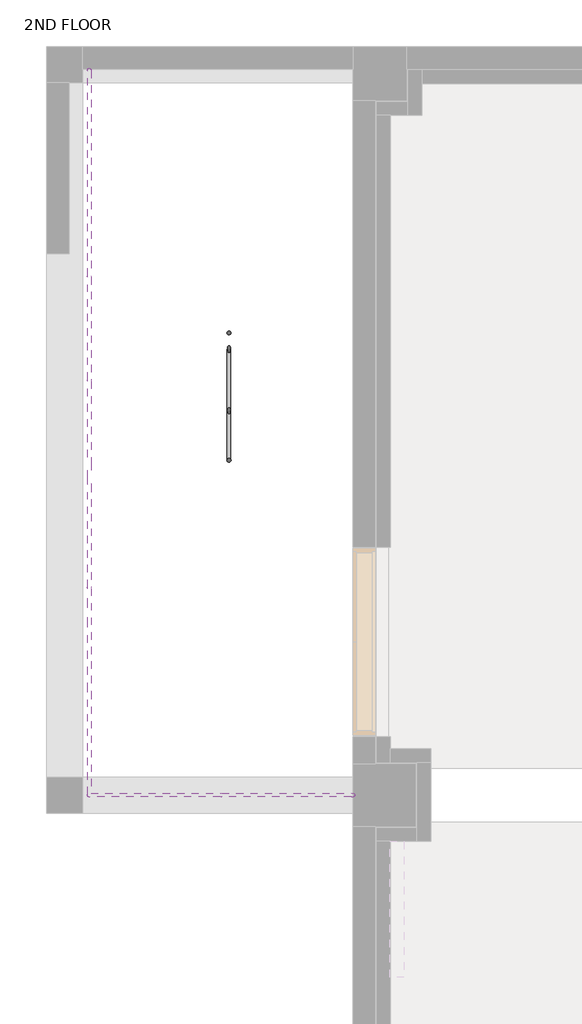
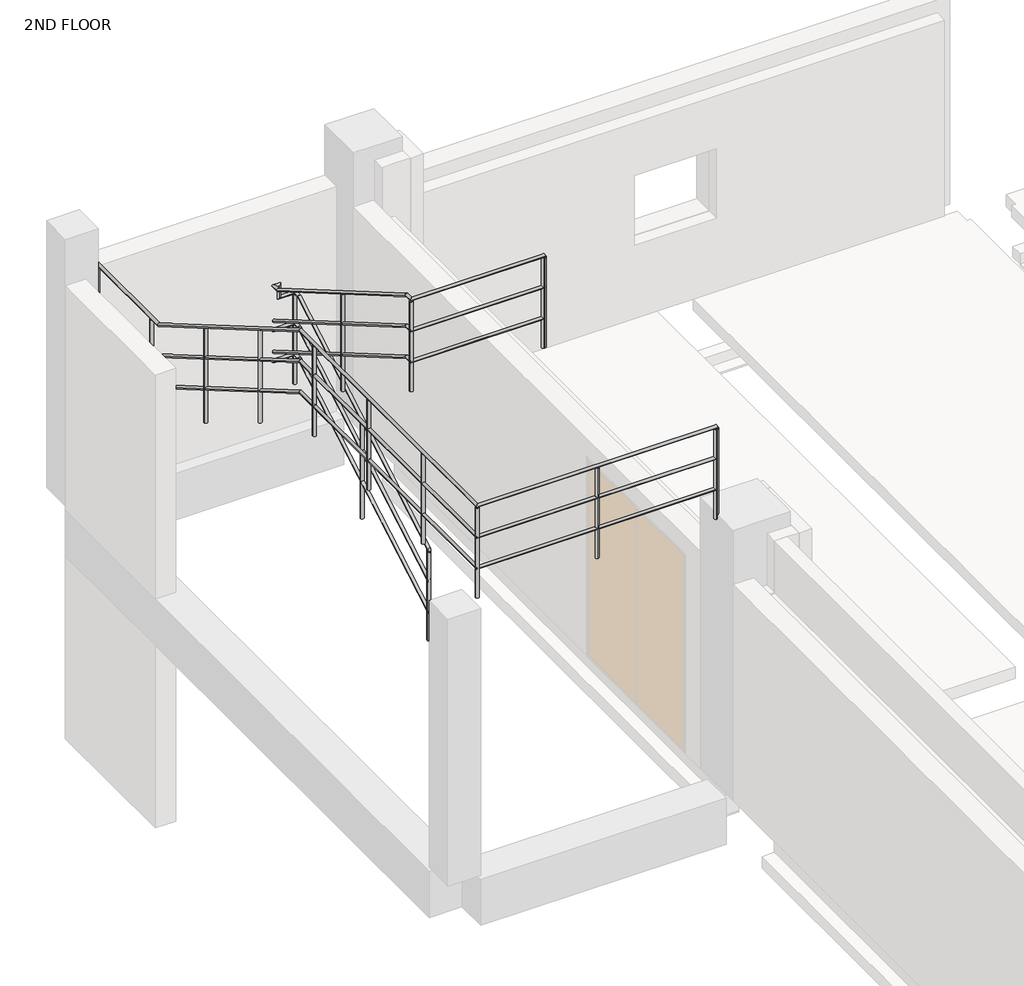
# One storey, part 6 of 7: 2 railings.
"""IFC4 building model written with IfcOpenShell, lengths in millimetres."""

from ifc_helpers import new_model, si_unit, point, frame, frame_2d, origin, place, context, project, spatial, circle_curve, ellipse_curve, trimmed, segment, composite_curve, outline, extrude, element, save
from ifc_brep_helpers import plane_surface, cylinder_surface, advanced_brep

model = new_model("IFC4")

# Units and contexts
model_context = context("Model", 3, world=origin())
ifc_project = project(units=[si_unit("LENGTHUNIT", "METRE", prefix="MILLI")], contexts=[model_context])

# Site, building, storey
site = spatial("IfcSite", under=ifc_project)
building = spatial("IfcBuilding", under=site)
storey = spatial("IfcBuildingStorey", under=building, Name="2ND FLOOR", Elevation=10600.0)

# Railings
placement = place(None, origin())
element("IfcRailing", 1, ObjectType="H_RL_AR_S10_Steel Handrail_H1200_STAIR", at=placement, inside=storey, context=model_context, shape_type="SolidModel", body=[
    advanced_brep(
    [(-1656.0, -4300.0, 11873.8369637), (-1694.0, -4300.0, 11873.8369637), (-1656.0, -1544.8633663, 13481.0), (-1694.0, -1544.8633663, 13481.0), (-1906.0, -1531.1366337, 13642.0), (-1944.0, -1531.1366337, 13642.0), (-1944.0, -4255.1366337, 15231.0), (-1906.0, -4255.1366337, 15231.0), (-1656.0, -1431.0, 13481.0), (-1694.0, -1469.0, 13481.0), (-1868.0, -1431.0, 13481.0), (-1868.0, -1469.0, 13481.0), (-1868.0, -1431.0, 13642.0), (-1868.0, -1469.0, 13642.0), (-1944.0, -1431.0, 13642.0), (-1906.0, -1469.0, 13642.0), (-1944.0, -4369.0, 15231.0), (-1906.0, -4331.0, 15231.0), (-300.0, -4369.0, 15231.0), (-300.0, -4331.0, 15231.0)],
    [
        (0, 1, ellipse_curve(frame((-1675.0, -4300.0, 11873.8369637), z_axis=(0.0, -1.0, 0.0), x_axis=(0.0, 0.0, -1.0)), 21.9963696, 19.0)),
        (1, 0, ellipse_curve(frame((-1675.0, -4300.0, 11873.8369637), z_axis=(0.0, -1.0, 0.0), x_axis=(0.0, 0.0, -1.0)), 21.9963696, 19.0)),
        (0, 2),
        (2, 3, ellipse_curve(frame((-1675.0, -1544.8633663, 13481.0), z_axis=(0.0, -0.9653442134540491, -0.2609799792144664), x_axis=(0.0, 0.2609799792144666, -0.9653442134540492)), 19.6820986, 19.0)),
        (3, 1),
        (3, 2, ellipse_curve(frame((-1675.0, -1544.8633663, 13481.0), z_axis=(0.0, -0.9653442134540491, -0.2609799792144664), x_axis=(0.0, 0.2609799792144666, -0.9653442134540492)), 19.6820986, 19.0)),
        (4, 5, ellipse_curve(frame((-1925.0, -1531.1366337, 13642.0), z_axis=(0.0, -0.965344213454049, 0.26097997921446664), x_axis=(0.0, -0.2609799792144667, -0.9653442134540489)), 19.6820986, 19.0)),
        (5, 6),
        (6, 7, ellipse_curve(frame((-1925.0, -4255.1366337, 15231.0), z_axis=(0.0, 0.965344213454049, -0.2609799792144667), x_axis=(0.0, -0.26097997921446675, -0.965344213454049)), 19.6820986, 19.0)),
        (7, 4),
        (5, 4, ellipse_curve(frame((-1925.0, -1531.1366337, 13642.0), z_axis=(0.0, -0.965344213454049, 0.26097997921446664), x_axis=(0.0, -0.2609799792144667, -0.9653442134540489)), 19.6820986, 19.0)),
        (7, 6, ellipse_curve(frame((-1925.0, -4255.1366337, 15231.0), z_axis=(0.0, 0.965344213454049, -0.2609799792144667), x_axis=(0.0, -0.26097997921446675, -0.965344213454049)), 19.6820986, 19.0)),
        (2, 8),
        (8, 9, ellipse_curve(frame((-1675.0, -1450.0, 13481.0), z_axis=(0.7071067811865466, -0.7071067811865485, 0.0), x_axis=(-0.7071067811865485, -0.7071067811865466, 0.0)), 26.8700577, 19.0)),
        (9, 3),
        (9, 8, ellipse_curve(frame((-1675.0, -1450.0, 13481.0), z_axis=(0.7071067811865466, -0.7071067811865485, 0.0), x_axis=(-0.7071067811865485, -0.7071067811865466, 0.0)), 26.8700577, 19.0)),
        (8, 10),
        (10, 11, ellipse_curve(frame((-1868.0, -1450.0, 13481.0), z_axis=(0.7071067811865475, 0.0, -0.7071067811865475), x_axis=(0.7071067811865476, 0.0, 0.7071067811865474)), 26.8700577, 19.0)),
        (11, 9),
        (11, 10, ellipse_curve(frame((-1868.0, -1450.0, 13481.0), z_axis=(0.7071067811865475, 0.0, -0.7071067811865475), x_axis=(0.7071067811865476, 0.0, 0.7071067811865474)), 26.8700577, 19.0)),
        (10, 12),
        (12, 13, ellipse_curve(frame((-1868.0, -1450.0, 13642.0), z_axis=(0.7071067811865475, 0.0, -0.7071067811865475), x_axis=(-0.7071067811865474, 0.0, -0.7071067811865476)), 26.8700577, 19.0)),
        (13, 11),
        (13, 12, ellipse_curve(frame((-1868.0, -1450.0, 13642.0), z_axis=(0.7071067811865475, 0.0, -0.7071067811865475), x_axis=(-0.7071067811865474, 0.0, -0.7071067811865476)), 26.8700577, 19.0)),
        (12, 14),
        (14, 15, ellipse_curve(frame((-1925.0, -1450.0, 13642.0), z_axis=(0.7071067811865416, 0.7071067811865536, 0.0), x_axis=(0.7071067811865535, -0.7071067811865417, 0.0)), 26.8700577, 19.0)),
        (15, 13),
        (15, 14, ellipse_curve(frame((-1925.0, -1450.0, 13642.0), z_axis=(0.7071067811865416, 0.7071067811865536, 0.0), x_axis=(0.7071067811865535, -0.7071067811865417, 0.0)), 26.8700577, 19.0)),
        (14, 5),
        (4, 15),
        (6, 16),
        (16, 17, ellipse_curve(frame((-1925.0, -4350.0, 15231.0), z_axis=(-0.7071067811865553, 0.7071067811865396, 0.0), x_axis=(0.7071067811865394, 0.7071067811865556, 0.0)), 26.8700577, 19.0)),
        (17, 7),
        (17, 16, ellipse_curve(frame((-1925.0, -4350.0, 15231.0), z_axis=(-0.7071067811865553, 0.7071067811865396, 0.0), x_axis=(0.7071067811865394, 0.7071067811865556, 0.0)), 26.8700577, 19.0)),
        (18, 19, circle_curve(frame((-300.0, -4350.0, 15231.0), z_axis=(1.0, 0.0, 0.0), x_axis=(0.0, 1.0, 0.0)), 19.0)),
        (19, 18, circle_curve(frame((-300.0, -4350.0, 15231.0), z_axis=(1.0, 0.0, 0.0), x_axis=(0.0, 1.0, 0.0)), 19.0)),
        (16, 18),
        (19, 17),
    ],
    [
        plane_surface(frame((-1675.0, -4300.0, 11895.8333333), z_axis=(0.0, -1.0, 0.0), x_axis=(0.0, 0.0, 1.0))),
        cylinder_surface(frame((-1675.0, -4290.4264505, 11879.4215342), z_axis=(0.0, -0.8637789008984333, -0.5038710255240862), x_axis=(-1.0, 0.0, 0.0)), 19.0),
        cylinder_surface(frame((-1925.0, -1535.5735495, 13644.5882009), z_axis=(0.0, 0.8637789008984331, -0.5038710255240867), x_axis=(1.0, 0.0, 0.0)), 19.0),
        cylinder_surface(frame((-1675.0, -1550.0, 13481.0), z_axis=(0.0, -1.0, 0.0), x_axis=(-1.0, 0.0, 0.0)), 19.0),
        cylinder_surface(frame((-1675.0, -1450.0, 13481.0), z_axis=(1.0, 0.0, 0.0), x_axis=(0.0, -1.0, 0.0)), 19.0),
        cylinder_surface(frame((-1868.0, -1450.0, 13500.0), z_axis=(0.0, 0.0, -1.0), x_axis=(0.0, -1.0, 0.0)), 19.0),
        cylinder_surface(frame((-1849.0, -1450.0, 13642.0), z_axis=(1.0, 0.0, 0.0), x_axis=(0.0, -1.0, 0.0)), 19.0),
        cylinder_surface(frame((-1925.0, -1450.0, 13642.0), z_axis=(0.0, 1.0, 0.0), x_axis=(1.0, 0.0, 0.0)), 19.0),
        cylinder_surface(frame((-1925.0, -4250.0, 15231.0), z_axis=(0.0, 1.0, 0.0), x_axis=(1.0, 0.0, 0.0)), 19.0),
        plane_surface(frame((-300.0, -4350.0, 15250.0), z_axis=(1.0, 0.0, 0.0), x_axis=(0.0, 1.0, 0.0))),
        cylinder_surface(frame((-1925.0, -4350.0, 15231.0), z_axis=(-1.0, 0.0, 0.0), x_axis=(0.0, 1.0, 0.0)), 19.0),
    ],
    [
        (0, [[1, 2]]),
        (1, [[-1, 3, 4, 5]]),
        (1, [[-2, -5, 6, -3]]),
        (2, [[7, 8, 9, 10]]),
        (2, [[11, -10, 12, -8]]),
        (3, [[-4, 13, 14, 15]]),
        (3, [[-6, -15, 16, -13]]),
        (4, [[-14, 17, 18, 19]]),
        (4, [[-16, -19, 20, -17]]),
        (5, [[-18, 21, 22, 23]]),
        (5, [[-20, -23, 24, -21]]),
        (6, [[-22, 25, 26, 27]]),
        (6, [[-24, -27, 28, -25]]),
        (7, [[-26, 29, -7, 30]]),
        (7, [[-28, -30, -11, -29]]),
        (8, [[-9, 31, 32, 33]]),
        (8, [[-12, -33, 34, -31]]),
        (9, [[35, 36]]),
        (10, [[-32, 37, -36, 38]]),
        (10, [[-34, -38, -35, -37]]),
    ],
),
    advanced_brep(
    [(-1656.0, -4300.0, 11073.8369637), (-1694.0, -4300.0, 11073.8369637), (-1656.0, -1544.8633663, 12681.0), (-1694.0, -1544.8633663, 12681.0), (-1656.0, -1431.0, 12681.0), (-1694.0, -1469.0, 12681.0)],
    [
        (0, 1, ellipse_curve(frame((-1675.0, -4300.0, 11073.8369637), z_axis=(0.0, -1.0, 0.0), x_axis=(0.0, 0.0, -1.0)), 21.9963696, 19.0)),
        (1, 0, ellipse_curve(frame((-1675.0, -4300.0, 11073.8369637), z_axis=(0.0, -1.0, 0.0), x_axis=(0.0, 0.0, -1.0)), 21.9963696, 19.0)),
        (0, 2),
        (2, 3, ellipse_curve(frame((-1675.0, -1544.8633663, 12681.0), z_axis=(0.0, -0.9653442134540491, -0.2609799792144664), x_axis=(0.0, 0.2609799792144666, -0.9653442134540492)), 19.6820986, 19.0)),
        (3, 1),
        (3, 2, ellipse_curve(frame((-1675.0, -1544.8633663, 12681.0), z_axis=(0.0, -0.9653442134540491, -0.2609799792144664), x_axis=(0.0, 0.2609799792144666, -0.9653442134540492)), 19.6820986, 19.0)),
        (4, 5, ellipse_curve(frame((-1675.0, -1450.0, 12681.0), z_axis=(-0.7071067811865455, 0.7071067811865496, 0.0), x_axis=(-0.7071067811865496, -0.7071067811865455, 0.0)), 26.8700577, 19.0)),
        (5, 4, ellipse_curve(frame((-1675.0, -1450.0, 12681.0), z_axis=(-0.7071067811865455, 0.7071067811865496, 0.0), x_axis=(-0.7071067811865496, -0.7071067811865455, 0.0)), 26.8700577, 19.0)),
        (2, 4),
        (5, 3),
    ],
    [
        plane_surface(frame((-1675.0, -4300.0, 11095.8333333), z_axis=(0.0, -1.0, 0.0), x_axis=(0.0, 0.0, 1.0))),
        cylinder_surface(frame((-1675.0, -4290.4264505, 11079.4215342), z_axis=(0.0, -0.8637789008984333, -0.5038710255240862), x_axis=(-1.0, 0.0, 0.0)), 19.0),
        plane_surface(frame((-1675.0, -1450.0, 12700.0), z_axis=(-0.7071067811865455, 0.7071067811865496, 0.0), x_axis=(0.7071067811865496, 0.7071067811865455, 0.0))),
        cylinder_surface(frame((-1675.0, -1550.0, 12681.0), z_axis=(0.0, -1.0, 0.0), x_axis=(-1.0, 0.0, 0.0)), 19.0),
    ],
    [
        (0, [[1, 2]]),
        (1, [[-1, 3, 4, 5]]),
        (1, [[-2, -5, 6, -3]]),
        (2, [[7, 8]]),
        (3, [[-4, 9, -8, 10]]),
        (3, [[-6, -10, -7, -9]]),
    ],
),
    advanced_brep(
    [(-1656.0, -1431.0, 12681.0), (-1694.0, -1469.0, 12681.0), (-1950.9853486, -1431.0, 12681.0), (-1918.1617504, -1469.0, 12681.0)],
    [
        (0, 1, ellipse_curve(frame((-1675.0, -1450.0, 12681.0), z_axis=(0.7071067811865455, -0.7071067811865496, 0.0), x_axis=(0.7071067811865496, 0.7071067811865455, 0.0)), 26.8700577, 19.0)),
        (1, 0, ellipse_curve(frame((-1675.0, -1450.0, 12681.0), z_axis=(0.7071067811865455, -0.7071067811865496, 0.0), x_axis=(0.7071067811865496, 0.7071067811865455, 0.0)), 26.8700577, 19.0)),
        (2, 3, ellipse_curve(frame((-1934.5735495, -1450.0, 12681.0), z_axis=(-0.707106781186549, -0.6107839182711431, 0.35629061899150194), x_axis=(0.707106781186546, -0.6107839182711456, 0.35629061899150344)), 26.8700577, 19.0)),
        (3, 2, ellipse_curve(frame((-1934.5735495, -1450.0, 12681.0), z_axis=(-0.707106781186549, -0.6107839182711431, 0.35629061899150194), x_axis=(0.707106781186546, -0.6107839182711456, 0.35629061899150344)), 26.8700577, 19.0)),
        (0, 2),
        (3, 1),
    ],
    [
        plane_surface(frame((-1675.0, -1450.0, 12700.0), z_axis=(0.7071067811865455, -0.7071067811865496, 0.0), x_axis=(0.7071067811865496, 0.7071067811865455, 0.0))),
        plane_surface(frame((-1925.0, -1450.0, 12700.0), z_axis=(-0.7071067811865491, -0.6107839182711432, 0.356290618991502), x_axis=(0.7071067811865461, -0.6107839182711456, 0.3562906189915033))),
        cylinder_surface(frame((-1675.0, -1450.0, 12681.0), z_axis=(1.0, 0.0, 0.0), x_axis=(0.0, -1.0, 0.0)), 19.0),
    ],
    [
        (0, [[1, 2]]),
        (1, [[3, 4]]),
        (2, [[-1, 5, -4, 6]]),
        (2, [[-2, -6, -3, -5]]),
    ],
),
    advanced_brep(
    [(-1944.0, -1443.1617504, 12790.6813181), (-1906.0, -1475.9853486, 12809.828417), (-1944.0, -4255.1366337, 14431.0), (-1906.0, -4255.1366337, 14431.0), (-1944.0, -4369.0, 14431.0), (-1906.0, -4331.0, 14431.0)],
    [
        (0, 1, ellipse_curve(frame((-1925.0, -1459.5735495, 12800.2548675), z_axis=(0.707106781186549, 0.6107839182711431, -0.35629061899150194), x_axis=(-0.7071067811865461, 0.6107839182711466, -0.3562906189915013)), 26.8700577, 19.0)),
        (1, 0, ellipse_curve(frame((-1925.0, -1459.5735495, 12800.2548675), z_axis=(0.707106781186549, 0.6107839182711431, -0.35629061899150194), x_axis=(-0.7071067811865461, 0.6107839182711466, -0.3562906189915013)), 26.8700577, 19.0)),
        (0, 2),
        (2, 3, ellipse_curve(frame((-1925.0, -4255.1366337, 14431.0), z_axis=(0.0, 0.965344213454049, -0.26097997921446664), x_axis=(0.0, -0.2609799792144663, -0.9653442134540491)), 19.6820986, 19.0)),
        (3, 1),
        (3, 2, ellipse_curve(frame((-1925.0, -4255.1366337, 14431.0), z_axis=(0.0, 0.965344213454049, -0.26097997921446664), x_axis=(0.0, -0.2609799792144663, -0.9653442134540491)), 19.6820986, 19.0)),
        (4, 5, ellipse_curve(frame((-1925.0, -4350.0, 14431.0), z_axis=(0.7071067811865476, -0.7071067811865475, 0.0), x_axis=(0.7071067811865475, 0.7071067811865476, 0.0)), 26.8700577, 19.0)),
        (5, 4, ellipse_curve(frame((-1925.0, -4350.0, 14431.0), z_axis=(0.7071067811865476, -0.7071067811865475, 0.0), x_axis=(0.7071067811865475, 0.7071067811865476, 0.0)), 26.8700577, 19.0)),
        (2, 4),
        (5, 3),
    ],
    [
        plane_surface(frame((-1925.0, -1450.0, 12816.6666667), z_axis=(0.7071067811865491, 0.6107839182711432, -0.356290618991502), x_axis=(0.7071067811865461, -0.6107839182711456, 0.3562906189915033))),
        cylinder_surface(frame((-1925.0, -1459.5735495, 12800.2548675), z_axis=(0.0, 0.8637789008984332, -0.5038710255240867), x_axis=(1.0, 0.0, 0.0)), 19.0),
        plane_surface(frame((-1925.0, -4350.0, 14450.0), z_axis=(0.7071067811865476, -0.7071067811865475, 0.0), x_axis=(0.7071067811865475, 0.7071067811865476, 0.0))),
        cylinder_surface(frame((-1925.0, -4250.0, 14431.0), z_axis=(0.0, 1.0, 0.0), x_axis=(1.0, 0.0, 0.0)), 19.0),
    ],
    [
        (0, [[1, 2]]),
        (1, [[-1, 3, 4, 5]]),
        (1, [[-2, -5, 6, -3]]),
        (2, [[7, 8]]),
        (3, [[-4, 9, -8, 10]]),
        (3, [[-6, -10, -7, -9]]),
    ],
),
    advanced_brep(
    [(-1656.0, -4300.0, 11473.8369637), (-1694.0, -4300.0, 11473.8369637), (-1656.0, -1544.8633663, 13081.0), (-1694.0, -1544.8633663, 13081.0), (-1656.0, -1431.0, 13081.0), (-1694.0, -1469.0, 13081.0)],
    [
        (0, 1, ellipse_curve(frame((-1675.0, -4300.0, 11473.8369637), z_axis=(0.0, -1.0, 0.0), x_axis=(0.0, 0.0, -1.0)), 21.9963696, 19.0)),
        (1, 0, ellipse_curve(frame((-1675.0, -4300.0, 11473.8369637), z_axis=(0.0, -1.0, 0.0), x_axis=(0.0, 0.0, -1.0)), 21.9963696, 19.0)),
        (0, 2),
        (2, 3, ellipse_curve(frame((-1675.0, -1544.8633663, 13081.0), z_axis=(0.0, -0.9653442134540491, -0.2609799792144664), x_axis=(0.0, 0.2609799792144666, -0.9653442134540492)), 19.6820986, 19.0)),
        (3, 1),
        (3, 2, ellipse_curve(frame((-1675.0, -1544.8633663, 13081.0), z_axis=(0.0, -0.9653442134540491, -0.2609799792144664), x_axis=(0.0, 0.2609799792144666, -0.9653442134540492)), 19.6820986, 19.0)),
        (4, 5, ellipse_curve(frame((-1675.0, -1450.0, 13081.0), z_axis=(-0.7071067811865455, 0.7071067811865496, 0.0), x_axis=(-0.7071067811865496, -0.7071067811865455, 0.0)), 26.8700577, 19.0)),
        (5, 4, ellipse_curve(frame((-1675.0, -1450.0, 13081.0), z_axis=(-0.7071067811865455, 0.7071067811865496, 0.0), x_axis=(-0.7071067811865496, -0.7071067811865455, 0.0)), 26.8700577, 19.0)),
        (2, 4),
        (5, 3),
    ],
    [
        plane_surface(frame((-1675.0, -4300.0, 11495.8333333), z_axis=(0.0, -1.0, 0.0), x_axis=(0.0, 0.0, 1.0))),
        cylinder_surface(frame((-1675.0, -4290.4264505, 11479.4215342), z_axis=(0.0, -0.8637789008984333, -0.5038710255240862), x_axis=(-1.0, 0.0, 0.0)), 19.0),
        plane_surface(frame((-1675.0, -1450.0, 13100.0), z_axis=(-0.7071067811865455, 0.7071067811865496, 0.0), x_axis=(0.7071067811865496, 0.7071067811865455, 0.0))),
        cylinder_surface(frame((-1675.0, -1550.0, 13081.0), z_axis=(0.0, -1.0, 0.0), x_axis=(-1.0, 0.0, 0.0)), 19.0),
    ],
    [
        (0, [[1, 2]]),
        (1, [[-1, 3, 4, 5]]),
        (1, [[-2, -5, 6, -3]]),
        (2, [[7, 8]]),
        (3, [[-4, 9, -8, 10]]),
        (3, [[-6, -10, -7, -9]]),
    ],
),
    advanced_brep(
    [(-1656.0, -1431.0, 13081.0), (-1694.0, -1469.0, 13081.0), (-1950.9853486, -1431.0, 13081.0), (-1918.1617504, -1469.0, 13081.0)],
    [
        (0, 1, ellipse_curve(frame((-1675.0, -1450.0, 13081.0), z_axis=(0.7071067811865455, -0.7071067811865496, 0.0), x_axis=(0.7071067811865496, 0.7071067811865455, 0.0)), 26.8700577, 19.0)),
        (1, 0, ellipse_curve(frame((-1675.0, -1450.0, 13081.0), z_axis=(0.7071067811865455, -0.7071067811865496, 0.0), x_axis=(0.7071067811865496, 0.7071067811865455, 0.0)), 26.8700577, 19.0)),
        (2, 3, ellipse_curve(frame((-1934.5735495, -1450.0, 13081.0), z_axis=(-0.707106781186549, -0.6107839182711431, 0.35629061899150194), x_axis=(0.707106781186546, -0.6107839182711456, 0.35629061899150344)), 26.8700577, 19.0)),
        (3, 2, ellipse_curve(frame((-1934.5735495, -1450.0, 13081.0), z_axis=(-0.707106781186549, -0.6107839182711431, 0.35629061899150194), x_axis=(0.707106781186546, -0.6107839182711456, 0.35629061899150344)), 26.8700577, 19.0)),
        (0, 2),
        (3, 1),
    ],
    [
        plane_surface(frame((-1675.0, -1450.0, 13100.0), z_axis=(0.7071067811865455, -0.7071067811865496, 0.0), x_axis=(0.7071067811865496, 0.7071067811865455, 0.0))),
        plane_surface(frame((-1925.0, -1450.0, 13100.0), z_axis=(-0.7071067811865491, -0.6107839182711432, 0.356290618991502), x_axis=(0.7071067811865461, -0.6107839182711456, 0.3562906189915033))),
        cylinder_surface(frame((-1675.0, -1450.0, 13081.0), z_axis=(1.0, 0.0, 0.0), x_axis=(0.0, -1.0, 0.0)), 19.0),
    ],
    [
        (0, [[1, 2]]),
        (1, [[3, 4]]),
        (2, [[-1, 5, -4, 6]]),
        (2, [[-2, -6, -3, -5]]),
    ],
),
    advanced_brep(
    [(-1944.0, -1443.1617504, 13190.6813181), (-1906.0, -1475.9853486, 13209.828417), (-1944.0, -4255.1366337, 14831.0), (-1906.0, -4255.1366337, 14831.0), (-1944.0, -4369.0, 14831.0), (-1906.0, -4331.0, 14831.0)],
    [
        (0, 1, ellipse_curve(frame((-1925.0, -1459.5735495, 13200.2548675), z_axis=(0.707106781186549, 0.6107839182711431, -0.35629061899150194), x_axis=(-0.7071067811865461, 0.6107839182711466, -0.3562906189915013)), 26.8700577, 19.0)),
        (1, 0, ellipse_curve(frame((-1925.0, -1459.5735495, 13200.2548675), z_axis=(0.707106781186549, 0.6107839182711431, -0.35629061899150194), x_axis=(-0.7071067811865461, 0.6107839182711466, -0.3562906189915013)), 26.8700577, 19.0)),
        (0, 2),
        (2, 3, ellipse_curve(frame((-1925.0, -4255.1366337, 14831.0), z_axis=(0.0, 0.965344213454049, -0.26097997921446664), x_axis=(0.0, -0.2609799792144663, -0.9653442134540491)), 19.6820986, 19.0)),
        (3, 1),
        (3, 2, ellipse_curve(frame((-1925.0, -4255.1366337, 14831.0), z_axis=(0.0, 0.965344213454049, -0.26097997921446664), x_axis=(0.0, -0.2609799792144663, -0.9653442134540491)), 19.6820986, 19.0)),
        (4, 5, ellipse_curve(frame((-1925.0, -4350.0, 14831.0), z_axis=(0.7071067811865476, -0.7071067811865475, 0.0), x_axis=(0.7071067811865475, 0.7071067811865476, 0.0)), 26.8700577, 19.0)),
        (5, 4, ellipse_curve(frame((-1925.0, -4350.0, 14831.0), z_axis=(0.7071067811865476, -0.7071067811865475, 0.0), x_axis=(0.7071067811865475, 0.7071067811865476, 0.0)), 26.8700577, 19.0)),
        (2, 4),
        (5, 3),
    ],
    [
        plane_surface(frame((-1925.0, -1450.0, 13216.6666667), z_axis=(0.7071067811865491, 0.6107839182711432, -0.356290618991502), x_axis=(0.7071067811865461, -0.6107839182711456, 0.3562906189915033))),
        cylinder_surface(frame((-1925.0, -1459.5735495, 13200.2548675), z_axis=(0.0, 0.8637789008984332, -0.5038710255240867), x_axis=(1.0, 0.0, 0.0)), 19.0),
        plane_surface(frame((-1925.0, -4350.0, 14850.0), z_axis=(0.7071067811865476, -0.7071067811865475, 0.0), x_axis=(0.7071067811865475, 0.7071067811865476, 0.0))),
        cylinder_surface(frame((-1925.0, -4250.0, 14831.0), z_axis=(0.0, 1.0, 0.0), x_axis=(1.0, 0.0, 0.0)), 19.0),
    ],
    [
        (0, [[1, 2]]),
        (1, [[-1, 3, 4, 5]]),
        (1, [[-2, -5, 6, -3]]),
        (2, [[7, 8]]),
        (3, [[-4, 9, -8, 10]]),
        (3, [[-6, -10, -7, -9]]),
    ],
),
    advanced_brep(
    [(-1944.0, -4369.0, 14431.0), (-1906.0, -4331.0, 14431.0), (-300.0, -4369.0, 14431.0), (-300.0, -4331.0, 14431.0)],
    [
        (0, 1, ellipse_curve(frame((-1925.0, -4350.0, 14431.0), z_axis=(-0.7071067811865476, 0.7071067811865475, 0.0), x_axis=(-0.7071067811865475, -0.7071067811865476, 0.0)), 26.8700577, 19.0)),
        (1, 0, ellipse_curve(frame((-1925.0, -4350.0, 14431.0), z_axis=(-0.7071067811865476, 0.7071067811865475, 0.0), x_axis=(-0.7071067811865475, -0.7071067811865476, 0.0)), 26.8700577, 19.0)),
        (2, 3, circle_curve(frame((-300.0, -4350.0, 14431.0), z_axis=(1.0, 0.0, 0.0), x_axis=(0.0, 1.0, 0.0)), 19.0)),
        (3, 2, circle_curve(frame((-300.0, -4350.0, 14431.0), z_axis=(1.0, 0.0, 0.0), x_axis=(0.0, 1.0, 0.0)), 19.0)),
        (0, 2),
        (3, 1),
    ],
    [
        plane_surface(frame((-1925.0, -4350.0, 14450.0), z_axis=(-0.7071067811865476, 0.7071067811865475, 0.0), x_axis=(0.7071067811865475, 0.7071067811865476, 0.0))),
        plane_surface(frame((-300.0, -4350.0, 14450.0), z_axis=(1.0, 0.0, 0.0), x_axis=(0.0, 1.0, 0.0))),
        cylinder_surface(frame((-1925.0, -4350.0, 14431.0), z_axis=(-1.0, 0.0, 0.0), x_axis=(0.0, 1.0, 0.0)), 19.0),
    ],
    [
        (0, [[1, 2]]),
        (1, [[3, 4]]),
        (2, [[-1, 5, -4, 6]]),
        (2, [[-2, -6, -3, -5]]),
    ],
),
    advanced_brep(
    [(-1944.0, -4369.0, 14831.0), (-1906.0, -4331.0, 14831.0), (-300.0, -4369.0, 14831.0), (-300.0, -4331.0, 14831.0)],
    [
        (0, 1, ellipse_curve(frame((-1925.0, -4350.0, 14831.0), z_axis=(-0.7071067811865476, 0.7071067811865475, 0.0), x_axis=(-0.7071067811865475, -0.7071067811865476, 0.0)), 26.8700577, 19.0)),
        (1, 0, ellipse_curve(frame((-1925.0, -4350.0, 14831.0), z_axis=(-0.7071067811865476, 0.7071067811865475, 0.0), x_axis=(-0.7071067811865475, -0.7071067811865476, 0.0)), 26.8700577, 19.0)),
        (2, 3, circle_curve(frame((-300.0, -4350.0, 14831.0), z_axis=(1.0, 0.0, 0.0), x_axis=(0.0, 1.0, 0.0)), 19.0)),
        (3, 2, circle_curve(frame((-300.0, -4350.0, 14831.0), z_axis=(1.0, 0.0, 0.0), x_axis=(0.0, 1.0, 0.0)), 19.0)),
        (0, 2),
        (3, 1),
    ],
    [
        plane_surface(frame((-1925.0, -4350.0, 14850.0), z_axis=(-0.7071067811865476, 0.7071067811865475, 0.0), x_axis=(0.7071067811865475, 0.7071067811865476, 0.0))),
        plane_surface(frame((-300.0, -4350.0, 14850.0), z_axis=(1.0, 0.0, 0.0), x_axis=(0.0, 1.0, 0.0))),
        cylinder_surface(frame((-1925.0, -4350.0, 14831.0), z_axis=(-1.0, 0.0, 0.0), x_axis=(0.0, 1.0, 0.0)), 19.0),
    ],
    [
        (0, [[1, 2]]),
        (1, [[3, 4]]),
        (2, [[-1, 5, -4, 6]]),
        (2, [[-2, -6, -3, -5]]),
    ],
),
    extrude(outline(composite_curve([segment(trimmed(circle_curve(frame_2d((-300.0, -4350.0)), 21.2), [point((-300.0, -4371.2))], [point((-300.0, -4328.8))], False, "CARTESIAN"), True, "CONTINUOUS"), segment(trimmed(circle_curve(frame_2d((-300.0, -4350.0)), 21.2), [point((-300.0, -4328.8))], [point((-300.0, -4371.2))], False, "CARTESIAN"), True, "CONTINUOUS")], self_intersect=False)), frame((0.0, 0.0, 14050.0), z_axis=(0.0, 0.0, 1.0), x_axis=(1.0, 0.0, 0.0)), (0.0, 0.0, 1.0), 1162.0),
    extrude(outline(composite_curve([segment(trimmed(circle_curve(frame_2d((-1925.0, -4350.0)), 21.2), [point((-1946.2, -4350.0))], [point((-1903.8, -4350.0))], False, "CARTESIAN"), True, "CONTINUOUS"), segment(trimmed(circle_curve(frame_2d((-1925.0, -4350.0)), 21.2), [point((-1903.8, -4350.0))], [point((-1946.2, -4350.0))], False, "CARTESIAN"), True, "CONTINUOUS")], self_intersect=False)), frame((0.0, 0.0, 14050.0), z_axis=(0.0, 0.0, 1.0), x_axis=(1.0, 0.0, 0.0)), (0.0, 0.0, 1.0), 1162.0),
    advanced_brep(
    [(-1903.8, -2900.0, 14418.5072607), (-1946.2, -2900.0, 14418.5072607), (-1946.2, -2900.0, 13175.0), (-1903.8, -2900.0, 13175.0)],
    [
        (0, 1, ellipse_curve(frame((-1925.0, -2900.0, 14418.5072607), z_axis=(0.0, -0.5038710255240875, -0.8637789008984328), x_axis=(0.0, -0.8637789008984329, 0.5038710255240872)), 24.5433177, 21.2)),
        (1, 2),
        (2, 3, circle_curve(frame((-1925.0, -2900.0, 13175.0), z_axis=(0.0, 0.0, 1.0), x_axis=(-1.0, 0.0, 0.0)), 21.2)),
        (3, 0),
        (3, 2, circle_curve(frame((-1925.0, -2900.0, 13175.0), z_axis=(0.0, 0.0, 1.0), x_axis=(-1.0, 0.0, 0.0)), 21.2)),
        (1, 0, ellipse_curve(frame((-1925.0, -2900.0, 14418.5072607), z_axis=(0.0, -0.5038710255240875, -0.8637789008984328), x_axis=(0.0, -0.8637789008984329, 0.5038710255240872)), 24.5433177, 21.2)),
    ],
    [
        cylinder_surface(frame((-1925.0, -2900.0, 13075.0), z_axis=(0.0, 0.0, 1.0), x_axis=(-1.0, 0.0, 0.0)), 21.2),
        plane_surface(frame((-1950.0, -2925.0, 14433.090594), z_axis=(0.0, 0.5038710255240875, 0.8637789008984328), x_axis=(1.0, 0.0, 0.0))),
        plane_surface(frame((-1950.0, -2875.0, 13175.0), z_axis=(0.0, 0.0, -1.0), x_axis=(1.0, 0.0, 0.0))),
    ],
    [
        (0, [[1, 2, 3, 4]]),
        (0, [[5, -2, 6, -4]]),
        (1, [[-6, -1]]),
        (2, [[-5, -3]]),
    ],
),
    extrude(outline(composite_curve([segment(trimmed(circle_curve(frame_2d((-1675.0, -1450.0)), 21.2), [point((-1653.8, -1450.0))], [point((-1696.2, -1450.0))], False, "CARTESIAN"), True, "CONTINUOUS"), segment(trimmed(circle_curve(frame_2d((-1675.0, -1450.0)), 21.2), [point((-1696.2, -1450.0))], [point((-1653.8, -1450.0))], False, "CARTESIAN"), True, "CONTINUOUS")], self_intersect=False)), frame((0.0, 0.0, 12300.0), z_axis=(0.0, 0.0, 1.0), x_axis=(1.0, 0.0, 0.0)), (0.0, 0.0, 1.0), 1162.0),
    advanced_brep(
    [(-1696.2, -2875.0, 12683.090594), (-1653.8, -2875.0, 12683.090594), (-1653.8, -2875.0, 11425.0), (-1696.2, -2875.0, 11425.0)],
    [
        (0, 1, ellipse_curve(frame((-1675.0, -2875.0, 12683.090594), z_axis=(0.0, 0.5038710255240839, -0.8637789008984348), x_axis=(0.0, 0.8637789008984348, 0.5038710255240838)), 24.5433177, 21.2)),
        (1, 2),
        (2, 3, circle_curve(frame((-1675.0, -2875.0, 11425.0), z_axis=(0.0, 0.0, 1.0), x_axis=(1.0, 0.0, 0.0)), 21.2)),
        (3, 0),
        (3, 2, circle_curve(frame((-1675.0, -2875.0, 11425.0), z_axis=(0.0, 0.0, 1.0), x_axis=(1.0, 0.0, 0.0)), 21.2)),
        (1, 0, ellipse_curve(frame((-1675.0, -2875.0, 12683.090594), z_axis=(0.0, 0.5038710255240839, -0.8637789008984348), x_axis=(0.0, 0.8637789008984348, 0.5038710255240838)), 24.5433177, 21.2)),
    ],
    [
        cylinder_surface(frame((-1675.0, -2875.0, 11325.0), z_axis=(0.0, 0.0, 1.0), x_axis=(1.0, 0.0, 0.0)), 21.2),
        plane_surface(frame((-1650.0, -2850.0, 12697.6739274), z_axis=(0.0, -0.5038710255240839, 0.8637789008984348), x_axis=(-1.0, 0.0, 0.0))),
        plane_surface(frame((-1650.0, -2900.0, 11425.0), z_axis=(0.0, 0.0, -1.0), x_axis=(-1.0, 0.0, 0.0))),
    ],
    [
        (0, [[1, 2, 3, 4]]),
        (0, [[5, -2, 6, -4]]),
        (1, [[-6, -1]]),
        (2, [[-5, -3]]),
    ],
),
    extrude(outline(composite_curve([segment(trimmed(circle_curve(frame_2d((-312.5, -4350.0)), 21.2), [point((-312.5, -4371.2))], [point((-312.5, -4328.8))], False, "CARTESIAN"), True, "CONTINUOUS"), segment(trimmed(circle_curve(frame_2d((-312.5, -4350.0)), 21.2), [point((-312.5, -4328.8))], [point((-312.5, -4371.2))], False, "CARTESIAN"), True, "CONTINUOUS")], self_intersect=False)), frame((0.0, 0.0, 14050.0), z_axis=(0.0, 0.0, 1.0), x_axis=(1.0, 0.0, 0.0)), (0.0, 0.0, 1.0), 1162.0),
    advanced_brep(
    [(-1696.2, -4287.5, 11859.1322607), (-1653.8, -4287.5, 11859.1322607), (-1653.8, -4287.5, 10703.125), (-1696.2, -4287.5, 10703.125)],
    [
        (0, 1, ellipse_curve(frame((-1675.0, -4287.5, 11859.1322607), z_axis=(0.0, 0.5038710255240857, -0.8637789008984338), x_axis=(0.0, 0.8637789008984338, 0.5038710255240854)), 24.5433177, 21.2)),
        (1, 2),
        (2, 3, circle_curve(frame((-1675.0, -4287.5, 10703.125), z_axis=(0.0, 0.0, 1.0), x_axis=(1.0, 0.0, 0.0)), 21.2)),
        (3, 0),
        (3, 2, circle_curve(frame((-1675.0, -4287.5, 10703.125), z_axis=(0.0, 0.0, 1.0), x_axis=(1.0, 0.0, 0.0)), 21.2)),
        (1, 0, ellipse_curve(frame((-1675.0, -4287.5, 11859.1322607), z_axis=(0.0, 0.5038710255240857, -0.8637789008984338), x_axis=(0.0, 0.8637789008984338, 0.5038710255240854)), 24.5433177, 21.2)),
    ],
    [
        cylinder_surface(frame((-1675.0, -4287.5, 10603.125), z_axis=(0.0, 0.0, 1.0), x_axis=(1.0, 0.0, 0.0)), 21.2),
        plane_surface(frame((-1650.0, -4262.5, 11873.715594), z_axis=(0.0, -0.5038710255240857, 0.8637789008984338), x_axis=(-1.0, 0.0, 0.0))),
        plane_surface(frame((-1650.0, -4312.5, 10703.125), z_axis=(0.0, 0.0, -1.0), x_axis=(-1.0, 0.0, 0.0))),
    ],
    [
        (0, [[1, 2, 3, 4]]),
        (0, [[5, -2, 6, -4]]),
        (1, [[-6, -1]]),
        (2, [[-5, -3]]),
    ],
),
])
element("IfcRailing", 2, ObjectType="H_RL_AR_S10_Steel Handrail_H1200_STAIR", at=placement, inside=storey, context=model_context, shape_type="SolidModel", body=[
    advanced_brep(
    [(-3244.0, 50.0, 13481.0), (-3206.0, 50.0, 13481.0), (-3244.0, -1255.1366337, 13481.0), (-3206.0, -1255.1366337, 13481.0), (-300.0, -8019.0, 15231.0), (-300.0, -7981.0, 15231.0), (-3206.0, -7981.0, 15231.0), (-3244.0, -8019.0, 15231.0), (-3244.0, -4255.1366337, 15231.0), (-3206.0, -4255.1366337, 15231.0)],
    [
        (0, 1, circle_curve(frame((-3225.0, 50.0, 13481.0), z_axis=(0.0, 1.0, 0.0), x_axis=(1.0, 0.0, 0.0)), 19.0)),
        (1, 0, circle_curve(frame((-3225.0, 50.0, 13481.0), z_axis=(0.0, 1.0, 0.0), x_axis=(1.0, 0.0, 0.0)), 19.0)),
        (0, 2),
        (2, 3, ellipse_curve(frame((-3225.0, -1255.1366337, 13481.0), z_axis=(0.0, 0.965344213454049, -0.26097997921446664), x_axis=(0.0, 0.2609799792144671, 0.965344213454049)), 19.6820986, 19.0)),
        (3, 1),
        (3, 2, ellipse_curve(frame((-3225.0, -1255.1366337, 13481.0), z_axis=(0.0, 0.965344213454049, -0.26097997921446664), x_axis=(0.0, 0.2609799792144671, 0.965344213454049)), 19.6820986, 19.0)),
        (4, 5, circle_curve(frame((-300.0, -8000.0, 15231.0), z_axis=(1.0, 0.0, 0.0), x_axis=(0.0, 1.0, 0.0)), 19.0)),
        (5, 4, circle_curve(frame((-300.0, -8000.0, 15231.0), z_axis=(1.0, 0.0, 0.0), x_axis=(0.0, 1.0, 0.0)), 19.0)),
        (6, 7, ellipse_curve(frame((-3225.0, -8000.0, 15231.0), z_axis=(0.7071067811865469, -0.7071067811865481, 0.0), x_axis=(-0.7071067811865481, -0.7071067811865469, 0.0)), 26.8700577, 19.0)),
        (7, 4),
        (5, 6),
        (7, 6, ellipse_curve(frame((-3225.0, -8000.0, 15231.0), z_axis=(0.7071067811865469, -0.7071067811865481, 0.0), x_axis=(-0.7071067811865481, -0.7071067811865469, 0.0)), 26.8700577, 19.0)),
        (2, 8),
        (8, 9, ellipse_curve(frame((-3225.0, -4255.1366337, 15231.0), z_axis=(0.0, 0.965344213454049, -0.2609799792144667), x_axis=(0.0, -0.26097997921446675, -0.965344213454049)), 19.6820986, 19.0)),
        (9, 3),
        (9, 8, ellipse_curve(frame((-3225.0, -4255.1366337, 15231.0), z_axis=(0.0, 0.965344213454049, -0.2609799792144667), x_axis=(0.0, -0.26097997921446675, -0.965344213454049)), 19.6820986, 19.0)),
        (8, 7),
        (6, 9),
    ],
    [
        plane_surface(frame((-3225.0, 50.0, 13500.0), z_axis=(0.0, 1.0, 0.0), x_axis=(0.0, 0.0, -1.0))),
        cylinder_surface(frame((-3225.0, 50.0, 13481.0), z_axis=(0.0, 1.0, 0.0), x_axis=(1.0, 0.0, 0.0)), 19.0),
        plane_surface(frame((-300.0, -8000.0, 15250.0), z_axis=(1.0, 0.0, 0.0), x_axis=(0.0, 1.0, 0.0))),
        cylinder_surface(frame((-3225.0, -8000.0, 15231.0), z_axis=(-1.0, 0.0, 0.0), x_axis=(0.0, 1.0, 0.0)), 19.0),
        cylinder_surface(frame((-3225.0, -1259.5735495, 13483.5882009), z_axis=(0.0, 0.8637789008984331, -0.5038710255240867), x_axis=(1.0, 0.0, 0.0)), 19.0),
        cylinder_surface(frame((-3225.0, -4250.0, 15231.0), z_axis=(0.0, 1.0, 0.0), x_axis=(1.0, 0.0, 0.0)), 19.0),
    ],
    [
        (0, [[1, 2]]),
        (1, [[-1, 3, 4, 5]]),
        (1, [[-2, -5, 6, -3]]),
        (2, [[7, 8]]),
        (3, [[9, 10, -8, 11]]),
        (3, [[12, -11, -7, -10]]),
        (4, [[-4, 13, 14, 15]]),
        (4, [[-6, -15, 16, -13]]),
        (5, [[-14, 17, -9, 18]]),
        (5, [[-16, -18, -12, -17]]),
    ],
),
    advanced_brep(
    [(-3206.0, 50.0, 12681.0), (-3244.0, 50.0, 12681.0), (-3206.0, -1255.1366337, 12681.0), (-3244.0, -1255.1366337, 12681.0), (-3206.0, -4255.1366337, 14431.0), (-3244.0, -4255.1366337, 14431.0), (-3206.0, -7981.0, 14431.0), (-3244.0, -8019.0, 14431.0)],
    [
        (0, 1, circle_curve(frame((-3225.0, 50.0, 12681.0), z_axis=(0.0, 1.0, 0.0), x_axis=(-1.0, 0.0, 0.0)), 19.0)),
        (1, 0, circle_curve(frame((-3225.0, 50.0, 12681.0), z_axis=(0.0, 1.0, 0.0), x_axis=(-1.0, 0.0, 0.0)), 19.0)),
        (0, 2),
        (2, 3, ellipse_curve(frame((-3225.0, -1255.1366337, 12681.0), z_axis=(0.0, 0.965344213454049, -0.26097997921446664), x_axis=(0.0, 0.2609799792144671, 0.965344213454049)), 19.6820986, 19.0)),
        (3, 1),
        (3, 2, ellipse_curve(frame((-3225.0, -1255.1366337, 12681.0), z_axis=(0.0, 0.965344213454049, -0.26097997921446664), x_axis=(0.0, 0.2609799792144671, 0.965344213454049)), 19.6820986, 19.0)),
        (2, 4),
        (4, 5, ellipse_curve(frame((-3225.0, -4255.1366337, 14431.0), z_axis=(0.0, 0.965344213454049, -0.2609799792144667), x_axis=(0.0, -0.26097997921446675, -0.965344213454049)), 19.6820986, 19.0)),
        (5, 3),
        (5, 4, ellipse_curve(frame((-3225.0, -4255.1366337, 14431.0), z_axis=(0.0, 0.965344213454049, -0.2609799792144667), x_axis=(0.0, -0.26097997921446675, -0.965344213454049)), 19.6820986, 19.0)),
        (6, 7, ellipse_curve(frame((-3225.0, -8000.0, 14431.0), z_axis=(0.7071067811865464, -0.7071067811865487, 0.0), x_axis=(0.7071067811865487, 0.7071067811865464, 0.0)), 26.8700577, 19.0)),
        (7, 6, ellipse_curve(frame((-3225.0, -8000.0, 14431.0), z_axis=(0.7071067811865464, -0.7071067811865487, 0.0), x_axis=(0.7071067811865487, 0.7071067811865464, 0.0)), 26.8700577, 19.0)),
        (4, 6),
        (7, 5),
    ],
    [
        plane_surface(frame((-3225.0, 50.0, 12700.0), z_axis=(0.0, 1.0, 0.0), x_axis=(0.0, 0.0, -1.0))),
        cylinder_surface(frame((-3225.0, 50.0, 12681.0), z_axis=(0.0, 1.0, 0.0), x_axis=(-1.0, 0.0, 0.0)), 19.0),
        cylinder_surface(frame((-3225.0, -1259.5735495, 12683.5882009), z_axis=(0.0, 0.8637789008984331, -0.5038710255240867), x_axis=(-1.0, 0.0, 0.0)), 19.0),
        plane_surface(frame((-3225.0, -8000.0, 14450.0), z_axis=(0.7071067811865464, -0.7071067811865487, 0.0), x_axis=(0.7071067811865487, 0.7071067811865464, 0.0))),
        cylinder_surface(frame((-3225.0, -4250.0, 14431.0), z_axis=(0.0, 1.0, 0.0), x_axis=(-1.0, 0.0, 0.0)), 19.0),
    ],
    [
        (0, [[1, 2]]),
        (1, [[-1, 3, 4, 5]]),
        (1, [[-2, -5, 6, -3]]),
        (2, [[-4, 7, 8, 9]]),
        (2, [[-6, -9, 10, -7]]),
        (3, [[11, 12]]),
        (4, [[-8, 13, -12, 14]]),
        (4, [[-10, -14, -11, -13]]),
    ],
),
    advanced_brep(
    [(-3206.0, -7981.0, 14431.0), (-3244.0, -8019.0, 14431.0), (-300.0, -7981.0, 14431.0), (-300.0, -8019.0, 14431.0)],
    [
        (0, 1, ellipse_curve(frame((-3225.0, -8000.0, 14431.0), z_axis=(-0.7071067811865464, 0.7071067811865487, 0.0), x_axis=(-0.7071067811865487, -0.7071067811865464, 0.0)), 26.8700577, 19.0)),
        (1, 0, ellipse_curve(frame((-3225.0, -8000.0, 14431.0), z_axis=(-0.7071067811865464, 0.7071067811865487, 0.0), x_axis=(-0.7071067811865487, -0.7071067811865464, 0.0)), 26.8700577, 19.0)),
        (2, 3, circle_curve(frame((-300.0, -8000.0, 14431.0), z_axis=(1.0, 0.0, 0.0), x_axis=(0.0, -1.0, 0.0)), 19.0)),
        (3, 2, circle_curve(frame((-300.0, -8000.0, 14431.0), z_axis=(1.0, 0.0, 0.0), x_axis=(0.0, -1.0, 0.0)), 19.0)),
        (0, 2),
        (3, 1),
    ],
    [
        plane_surface(frame((-3225.0, -8000.0, 14450.0), z_axis=(-0.7071067811865464, 0.7071067811865487, 0.0), x_axis=(0.7071067811865487, 0.7071067811865464, 0.0))),
        plane_surface(frame((-300.0, -8000.0, 14450.0), z_axis=(1.0, 0.0, 0.0), x_axis=(0.0, 1.0, 0.0))),
        cylinder_surface(frame((-3225.0, -8000.0, 14431.0), z_axis=(-1.0, 0.0, 0.0), x_axis=(0.0, -1.0, 0.0)), 19.0),
    ],
    [
        (0, [[1, 2]]),
        (1, [[3, 4]]),
        (2, [[-1, 5, -4, 6]]),
        (2, [[-2, -6, -3, -5]]),
    ],
),
    advanced_brep(
    [(-3206.0, 50.0, 13081.0), (-3244.0, 50.0, 13081.0), (-3206.0, -1255.1366337, 13081.0), (-3244.0, -1255.1366337, 13081.0), (-3206.0, -4255.1366337, 14831.0), (-3244.0, -4255.1366337, 14831.0), (-3206.0, -7981.0, 14831.0), (-3244.0, -8019.0, 14831.0)],
    [
        (0, 1, circle_curve(frame((-3225.0, 50.0, 13081.0), z_axis=(0.0, 1.0, 0.0), x_axis=(-1.0, 0.0, 0.0)), 19.0)),
        (1, 0, circle_curve(frame((-3225.0, 50.0, 13081.0), z_axis=(0.0, 1.0, 0.0), x_axis=(-1.0, 0.0, 0.0)), 19.0)),
        (0, 2),
        (2, 3, ellipse_curve(frame((-3225.0, -1255.1366337, 13081.0), z_axis=(0.0, 0.965344213454049, -0.26097997921446664), x_axis=(0.0, 0.2609799792144671, 0.965344213454049)), 19.6820986, 19.0)),
        (3, 1),
        (3, 2, ellipse_curve(frame((-3225.0, -1255.1366337, 13081.0), z_axis=(0.0, 0.965344213454049, -0.26097997921446664), x_axis=(0.0, 0.2609799792144671, 0.965344213454049)), 19.6820986, 19.0)),
        (2, 4),
        (4, 5, ellipse_curve(frame((-3225.0, -4255.1366337, 14831.0), z_axis=(0.0, 0.965344213454049, -0.2609799792144667), x_axis=(0.0, -0.26097997921446675, -0.965344213454049)), 19.6820986, 19.0)),
        (5, 3),
        (5, 4, ellipse_curve(frame((-3225.0, -4255.1366337, 14831.0), z_axis=(0.0, 0.965344213454049, -0.2609799792144667), x_axis=(0.0, -0.26097997921446675, -0.965344213454049)), 19.6820986, 19.0)),
        (6, 7, ellipse_curve(frame((-3225.0, -8000.0, 14831.0), z_axis=(0.7071067811865464, -0.7071067811865487, 0.0), x_axis=(0.7071067811865487, 0.7071067811865464, 0.0)), 26.8700577, 19.0)),
        (7, 6, ellipse_curve(frame((-3225.0, -8000.0, 14831.0), z_axis=(0.7071067811865464, -0.7071067811865487, 0.0), x_axis=(0.7071067811865487, 0.7071067811865464, 0.0)), 26.8700577, 19.0)),
        (4, 6),
        (7, 5),
    ],
    [
        plane_surface(frame((-3225.0, 50.0, 13100.0), z_axis=(0.0, 1.0, 0.0), x_axis=(0.0, 0.0, -1.0))),
        cylinder_surface(frame((-3225.0, 50.0, 13081.0), z_axis=(0.0, 1.0, 0.0), x_axis=(-1.0, 0.0, 0.0)), 19.0),
        cylinder_surface(frame((-3225.0, -1259.5735495, 13083.5882009), z_axis=(0.0, 0.8637789008984331, -0.5038710255240867), x_axis=(-1.0, 0.0, 0.0)), 19.0),
        plane_surface(frame((-3225.0, -8000.0, 14850.0), z_axis=(0.7071067811865464, -0.7071067811865487, 0.0), x_axis=(0.7071067811865487, 0.7071067811865464, 0.0))),
        cylinder_surface(frame((-3225.0, -4250.0, 14831.0), z_axis=(0.0, 1.0, 0.0), x_axis=(-1.0, 0.0, 0.0)), 19.0),
    ],
    [
        (0, [[1, 2]]),
        (1, [[-1, 3, 4, 5]]),
        (1, [[-2, -5, 6, -3]]),
        (2, [[-4, 7, 8, 9]]),
        (2, [[-6, -9, 10, -7]]),
        (3, [[11, 12]]),
        (4, [[-8, 13, -12, 14]]),
        (4, [[-10, -14, -11, -13]]),
    ],
),
    advanced_brep(
    [(-3206.0, -7981.0, 14831.0), (-3244.0, -8019.0, 14831.0), (-300.0, -7981.0, 14831.0), (-300.0, -8019.0, 14831.0)],
    [
        (0, 1, ellipse_curve(frame((-3225.0, -8000.0, 14831.0), z_axis=(-0.7071067811865464, 0.7071067811865487, 0.0), x_axis=(-0.7071067811865487, -0.7071067811865464, 0.0)), 26.8700577, 19.0)),
        (1, 0, ellipse_curve(frame((-3225.0, -8000.0, 14831.0), z_axis=(-0.7071067811865464, 0.7071067811865487, 0.0), x_axis=(-0.7071067811865487, -0.7071067811865464, 0.0)), 26.8700577, 19.0)),
        (2, 3, circle_curve(frame((-300.0, -8000.0, 14831.0), z_axis=(1.0, 0.0, 0.0), x_axis=(0.0, -1.0, 0.0)), 19.0)),
        (3, 2, circle_curve(frame((-300.0, -8000.0, 14831.0), z_axis=(1.0, 0.0, 0.0), x_axis=(0.0, -1.0, 0.0)), 19.0)),
        (0, 2),
        (3, 1),
    ],
    [
        plane_surface(frame((-3225.0, -8000.0, 14850.0), z_axis=(-0.7071067811865464, 0.7071067811865487, 0.0), x_axis=(0.7071067811865487, 0.7071067811865464, 0.0))),
        plane_surface(frame((-300.0, -8000.0, 14850.0), z_axis=(1.0, 0.0, 0.0), x_axis=(0.0, 1.0, 0.0))),
        cylinder_surface(frame((-3225.0, -8000.0, 14831.0), z_axis=(-1.0, 0.0, 0.0), x_axis=(0.0, -1.0, 0.0)), 19.0),
    ],
    [
        (0, [[1, 2]]),
        (1, [[3, 4]]),
        (2, [[-1, 5, -4, 6]]),
        (2, [[-2, -6, -3, -5]]),
    ],
),
    extrude(outline(composite_curve([segment(trimmed(circle_curve(frame_2d((-300.0, -8000.0)), 21.2), [point((-300.0, -7978.8))], [point((-300.0, -8021.2))], False, "CARTESIAN"), True, "CONTINUOUS"), segment(trimmed(circle_curve(frame_2d((-300.0, -8000.0)), 21.2), [point((-300.0, -8021.2))], [point((-300.0, -7978.8))], False, "CARTESIAN"), True, "CONTINUOUS")], self_intersect=False)), frame((0.0, 0.0, 14050.0), z_axis=(0.0, 0.0, 1.0), x_axis=(1.0, 0.0, 0.0)), (0.0, 0.0, 1.0), 1162.0),
    extrude(outline(composite_curve([segment(trimmed(circle_curve(frame_2d((-1762.5, -8000.0)), 21.2), [point((-1762.5, -7978.8))], [point((-1762.5, -8021.2))], False, "CARTESIAN"), True, "CONTINUOUS"), segment(trimmed(circle_curve(frame_2d((-1762.5, -8000.0)), 21.2), [point((-1762.5, -8021.2))], [point((-1762.5, -7978.8))], False, "CARTESIAN"), True, "CONTINUOUS")], self_intersect=False)), frame((0.0, 0.0, 14050.0), z_axis=(0.0, 0.0, 1.0), x_axis=(1.0, 0.0, 0.0)), (0.0, 0.0, 1.0), 1162.0),
    extrude(outline(composite_curve([segment(trimmed(circle_curve(frame_2d((-3225.0, -8000.0)), 21.2), [point((-3203.8, -8000.0))], [point((-3246.2, -8000.0))], False, "CARTESIAN"), True, "CONTINUOUS"), segment(trimmed(circle_curve(frame_2d((-3225.0, -8000.0)), 21.2), [point((-3246.2, -8000.0))], [point((-3203.8, -8000.0))], False, "CARTESIAN"), True, "CONTINUOUS")], self_intersect=False)), frame((0.0, 0.0, 14050.0), z_axis=(0.0, 0.0, 1.0), x_axis=(1.0, 0.0, 0.0)), (0.0, 0.0, 1.0), 1162.0),
    extrude(outline(composite_curve([segment(trimmed(circle_curve(frame_2d((-3225.0, -6850.0)), 21.2), [point((-3203.8, -6850.0))], [point((-3246.2, -6850.0))], False, "CARTESIAN"), True, "CONTINUOUS"), segment(trimmed(circle_curve(frame_2d((-3225.0, -6850.0)), 21.2), [point((-3246.2, -6850.0))], [point((-3203.8, -6850.0))], False, "CARTESIAN"), True, "CONTINUOUS")], self_intersect=False)), frame((0.0, 0.0, 14050.0), z_axis=(0.0, 0.0, 1.0), x_axis=(1.0, 0.0, 0.0)), (0.0, 0.0, 1.0), 1162.0),
    extrude(outline(composite_curve([segment(trimmed(circle_curve(frame_2d((-3225.0, -5700.0)), 21.2), [point((-3203.8, -5700.0))], [point((-3246.2, -5700.0))], False, "CARTESIAN"), True, "CONTINUOUS"), segment(trimmed(circle_curve(frame_2d((-3225.0, -5700.0)), 21.2), [point((-3246.2, -5700.0))], [point((-3203.8, -5700.0))], False, "CARTESIAN"), True, "CONTINUOUS")], self_intersect=False)), frame((0.0, 0.0, 14050.0), z_axis=(0.0, 0.0, 1.0), x_axis=(1.0, 0.0, 0.0)), (0.0, 0.0, 1.0), 1162.0),
    extrude(outline(composite_curve([segment(trimmed(circle_curve(frame_2d((-3225.0, -4550.0)), 21.2), [point((-3203.8, -4550.0))], [point((-3246.2, -4550.0))], False, "CARTESIAN"), True, "CONTINUOUS"), segment(trimmed(circle_curve(frame_2d((-3225.0, -4550.0)), 21.2), [point((-3246.2, -4550.0))], [point((-3203.8, -4550.0))], False, "CARTESIAN"), True, "CONTINUOUS")], self_intersect=False)), frame((0.0, 0.0, 14050.0), z_axis=(0.0, 0.0, 1.0), x_axis=(1.0, 0.0, 0.0)), (0.0, 0.0, 1.0), 1162.0),
    advanced_brep(
    [(-3246.2, -3400.0, 14710.1739274), (-3246.2, -3400.0, 13525.0), (-3203.8, -3400.0, 13525.0), (-3203.8, -3400.0, 14710.1739274)],
    [
        (0, 1),
        (1, 2, circle_curve(frame((-3225.0, -3400.0, 13525.0), z_axis=(0.0, 0.0, 1.0), x_axis=(1.0, 0.0, 0.0)), 21.2)),
        (2, 3),
        (3, 0, ellipse_curve(frame((-3225.0, -3400.0, 14710.1739274), z_axis=(0.0, -0.5038710255240875, -0.8637789008984328), x_axis=(0.0, -0.8637789008984329, 0.5038710255240872)), 24.5433177, 21.2)),
        (0, 3, ellipse_curve(frame((-3225.0, -3400.0, 14710.1739274), z_axis=(0.0, -0.5038710255240875, -0.8637789008984328), x_axis=(0.0, -0.8637789008984329, 0.5038710255240872)), 24.5433177, 21.2)),
        (2, 1, circle_curve(frame((-3225.0, -3400.0, 13525.0), z_axis=(0.0, 0.0, 1.0), x_axis=(1.0, 0.0, 0.0)), 21.2)),
    ],
    [
        cylinder_surface(frame((-3225.0, -3400.0, 13425.0), z_axis=(0.0, 0.0, 1.0), x_axis=(1.0, 0.0, 0.0)), 21.2),
        plane_surface(frame((-3200.0, -3425.0, 14724.7572607), z_axis=(0.0, 0.5038710255240875, 0.8637789008984328), x_axis=(-1.0, 0.0, 0.0))),
        plane_surface(frame((-3200.0, -3375.0, 13525.0), z_axis=(0.0, 0.0, -1.0), x_axis=(-1.0, 0.0, 0.0))),
    ],
    [
        (0, [[1, 2, 3, 4]]),
        (0, [[-1, 5, -3, 6]]),
        (1, [[-4, -5]]),
        (2, [[-2, -6]]),
    ],
),
    advanced_brep(
    [(-3246.2, -2250.0, 14039.340594), (-3246.2, -2250.0, 12825.0), (-3203.8, -2250.0, 12825.0), (-3203.8, -2250.0, 14039.340594)],
    [
        (0, 1),
        (1, 2, circle_curve(frame((-3225.0, -2250.0, 12825.0), z_axis=(0.0, 0.0, 1.0), x_axis=(1.0, 0.0, 0.0)), 21.2)),
        (2, 3),
        (3, 0, ellipse_curve(frame((-3225.0, -2250.0, 14039.340594), z_axis=(0.0, -0.5038710255240857, -0.8637789008984338), x_axis=(0.0, -0.8637789008984338, 0.5038710255240854)), 24.5433177, 21.2)),
        (0, 3, ellipse_curve(frame((-3225.0, -2250.0, 14039.340594), z_axis=(0.0, -0.5038710255240857, -0.8637789008984338), x_axis=(0.0, -0.8637789008984338, 0.5038710255240854)), 24.5433177, 21.2)),
        (2, 1, circle_curve(frame((-3225.0, -2250.0, 12825.0), z_axis=(0.0, 0.0, 1.0), x_axis=(1.0, 0.0, 0.0)), 21.2)),
    ],
    [
        cylinder_surface(frame((-3225.0, -2250.0, 12725.0), z_axis=(0.0, 0.0, 1.0), x_axis=(1.0, 0.0, 0.0)), 21.2),
        plane_surface(frame((-3200.0, -2275.0, 14053.9239274), z_axis=(0.0, 0.5038710255240857, 0.8637789008984338), x_axis=(-1.0, 0.0, 0.0))),
        plane_surface(frame((-3200.0, -2225.0, 12825.0), z_axis=(0.0, 0.0, -1.0), x_axis=(-1.0, 0.0, 0.0))),
    ],
    [
        (0, [[1, 2, 3, 4]]),
        (0, [[-1, 5, -3, 6]]),
        (1, [[-4, -5]]),
        (2, [[-2, -6]]),
    ],
),
    extrude(outline(composite_curve([segment(trimmed(circle_curve(frame_2d((-3225.0, -1100.0)), 21.2), [point((-3203.8, -1100.0))], [point((-3246.2, -1100.0))], False, "CARTESIAN"), True, "CONTINUOUS"), segment(trimmed(circle_curve(frame_2d((-3225.0, -1100.0)), 21.2), [point((-3246.2, -1100.0))], [point((-3203.8, -1100.0))], False, "CARTESIAN"), True, "CONTINUOUS")], self_intersect=False)), frame((0.0, 0.0, 12300.0), z_axis=(0.0, 0.0, 1.0), x_axis=(1.0, 0.0, 0.0)), (0.0, 0.0, 1.0), 1162.0),
    extrude(outline(composite_curve([segment(trimmed(circle_curve(frame_2d((-312.5, -8000.0)), 21.2), [point((-312.5, -7978.8))], [point((-312.5, -8021.2))], False, "CARTESIAN"), True, "CONTINUOUS"), segment(trimmed(circle_curve(frame_2d((-312.5, -8000.0)), 21.2), [point((-312.5, -8021.2))], [point((-312.5, -7978.8))], False, "CARTESIAN"), True, "CONTINUOUS")], self_intersect=False)), frame((0.0, 0.0, 14050.0), z_axis=(0.0, 0.0, 1.0), x_axis=(1.0, 0.0, 0.0)), (0.0, 0.0, 1.0), 1162.0),
    extrude(outline(composite_curve([segment(trimmed(circle_curve(frame_2d((-3225.0, 37.5)), 21.2), [point((-3203.8, 37.5))], [point((-3246.2, 37.5))], False, "CARTESIAN"), True, "CONTINUOUS"), segment(trimmed(circle_curve(frame_2d((-3225.0, 37.5)), 21.2), [point((-3246.2, 37.5))], [point((-3203.8, 37.5))], False, "CARTESIAN"), True, "CONTINUOUS")], self_intersect=False)), frame((0.0, 0.0, 12300.0), z_axis=(0.0, 0.0, 1.0), x_axis=(1.0, 0.0, 0.0)), (0.0, 0.0, 1.0), 1162.0),
])

save(model, "model.ifc")

# Revit data of these elements
# Type "H_RL_AR_S10_Steel Handrail_H1200_STAIR"
#   built-in parameter 1008612 = 0.166667 (stored number, unit not read)
#   built-in parameter 1008611 = 0.166667 (stored number, unit not read)
#   built-in parameter 1008609 = 0.459318 (stored number, unit not read)
#   built-in parameter 1008604 = 0.25 (stored number, unit not read)
#   built-in parameter 1008603 = 0.166667 (stored number, unit not read)
#   Railing Height = 1200 mm
#   built-in parameter 1008632 = 1
#   built-in parameter 1008610 = 1
#   built-in parameter 1008618 = M_Baluster - Square : 25mm
# Elements 1, 2 (IfcRailing, "H_RL_AR_S10_Steel Handrail_H1200_STAIR")
#   Phase Created = New Construction
